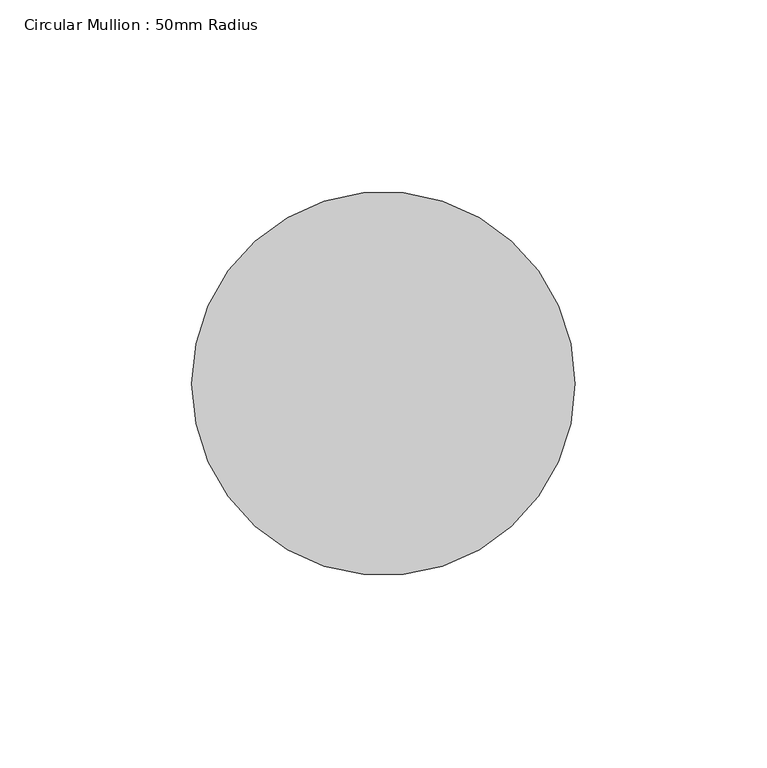
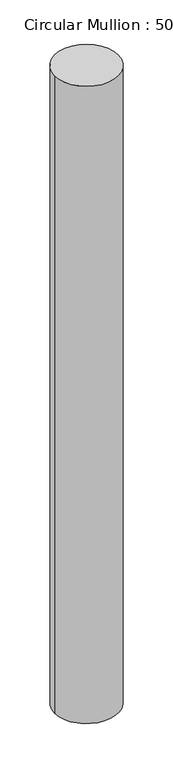
"""IFC4 building model written with IfcOpenShell, lengths in millimetres: member geometry, Circular Mullion : 50mm Radius."""

from ifc_helpers import new_model, si_unit, point, frame, origin, origin_2d, place, context, project, spatial, circle_curve, trimmed, segment, composite_curve, outline, extrude, source, transform, mapped, element, save


def circular_mullion_50mm_radius_2c407059(model_context):
    return source(origin(), model_context, "Body", "SweptSolid", [
        extrude(outline(composite_curve([segment(trimmed(circle_curve(origin_2d(), 50.0), [point((50.0, 0.0))], [point((-50.0, 0.0))], False, "CARTESIAN"), True, "CONTINUOUS"), segment(trimmed(circle_curve(origin_2d(), 50.0), [point((-50.0, 0.0))], [point((50.0, 0.0))], False, "CARTESIAN"), True, "CONTINUOUS")], self_intersect=False)), frame((0.0, 0.0, -1061.8482825), z_axis=(0.0, 0.0, 1.0), x_axis=(1.0, 0.0, 0.0)), (0.0, 0.0, 1.0), 1061.8482825),
    ])


if __name__ == "__main__":
    model = new_model("IFC4")
    model_context = context("Model", 3, world=origin())
    ifc_project = project(units=[si_unit("LENGTHUNIT", "METRE", prefix="MILLI")], contexts=[model_context])
    site = spatial("IfcSite", under=ifc_project)
    building = spatial("IfcBuilding", under=site)
    placement = place(None, origin())
    circular_mullion_50mm_radius_shape = circular_mullion_50mm_radius_2c407059(model_context)
    element("IfcMember", 1, ObjectType="Circular Mullion : 50mm Radius", at=placement, inside=building, context=model_context, shape_type="MappedRepresentation", body=[
        mapped(circular_mullion_50mm_radius_shape, transform((0.0, 0.0, 0.0), x_axis=(1.0, 0.0, 0.0), y_axis=(0.0, 1.0, 0.0), z_axis=(0.0, 0.0, 1.0))),
    ])
    save(model, "model.ifc")

# Revit data of these elements
# Type "Circular Mullion : 50mm Radius"
#   built-in parameter 1007350 = 0.164042 (stored number, unit not read)
# Element 1 (IfcMember, "Circular Mullion : 50mm Radius")
#   Materials on its faces: "Aluminium"
# Materials
#   "Aluminium": class "Metal", colour RGB 247 247 247, transparency 0, Description = "Aluminium 6061", Cost = 0
